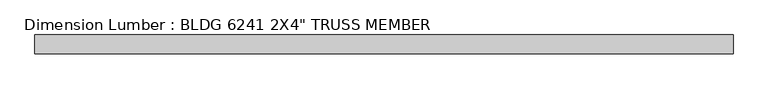
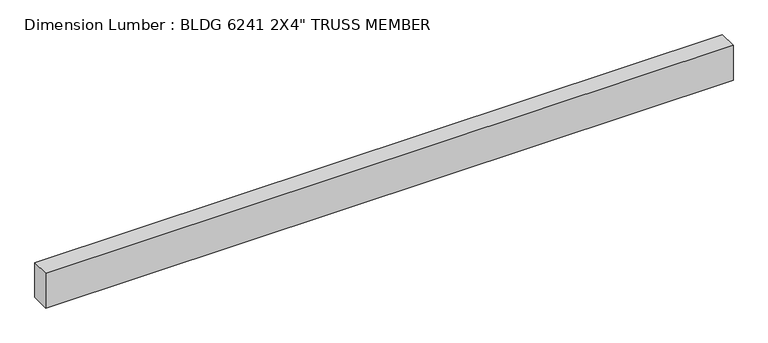
"""IFC4 building model written with IfcOpenShell, lengths in millimetres: beam geometry."""

from ifc_helpers import new_model, si_unit, frame, origin, place, context, project, spatial, polyline, outline, extrude, source, transform, mapped, element, save


def beam_a7f65a44(model_context):
    return source(origin(), model_context, "Body", "SweptSolid", [
        extrude(outline(polyline([(921.932951, 25.4), (921.932951, -25.4), (-972.7329504, -25.4), (-972.7329504, 25.4), (921.932951, 25.4)])), frame((0.0, 0.0, -50.8), z_axis=(0.0, 0.0, 1.0), x_axis=(1.0, 0.0, 0.0)), (0.0, 0.0, 1.0), 101.6),
    ])


if __name__ == "__main__":
    model = new_model("IFC4")
    model_context = context("Model", 3, world=origin())
    ifc_project = project(units=[si_unit("LENGTHUNIT", "METRE", prefix="MILLI")], contexts=[model_context])
    site = spatial("IfcSite", under=ifc_project)
    building = spatial("IfcBuilding", under=site)
    placement = place(None, origin())
    beam_shape = beam_a7f65a44(model_context)
    element("IfcBeam", 1, ObjectType="Dimension Lumber : BLDG 6241 2X4\" TRUSS MEMBER", at=placement, inside=building, context=model_context, shape_type="MappedRepresentation", body=[
        mapped(beam_shape, transform((0.0, 0.0, 0.0), x_axis=(1.0, 0.0, 0.0), y_axis=(0.0, 1.0, 0.0), z_axis=(0.0, 0.0, 1.0))),
    ])
    save(model, "model.ifc")

# Revit data of these elements
# Type "Dimension Lumber : BLDG 6241 2X4\" TRUSS MEMBER"
#   Assembly Code = "B10"
#   A = 0.273472 SF
#   Length [instance default] = 5' - 0"
#   b = 0' - 2"
#   d = 0' - 4"
#   Structural Material [instance default] = Softwood, Lumber
# Element 1 (IfcBeam, "Dimension Lumber : BLDG 6241 2X4\" TRUSS MEMBER")
#   Materials on its faces: "Softwood, Lumber"
# Materials
#   "Softwood, Lumber": class "Wood", colour RGB 223 192 134, transparency 0, Description = "Pinus Echinata", Cost = 0
